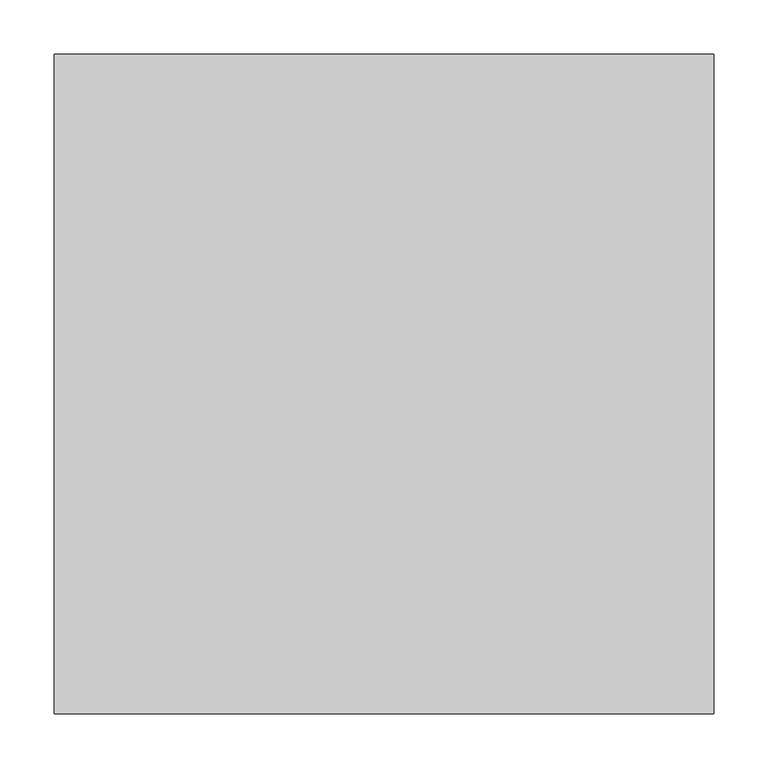
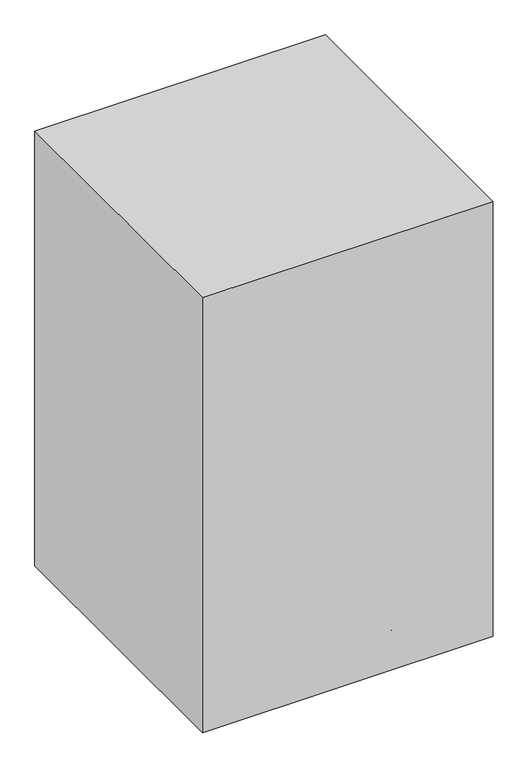
"""IFC4 building model written with IfcOpenShell, lengths in millimetres: proxy geometry, F0340 - Stool, Self Adjusting : F0340 - Stool, Self Adjusting."""

import ifcopenshell
import ifcopenshell.guid

model = None  # the IFC model being written
_history = None  # IfcOwnerHistory: only IFC2X3 demands one
_inside = {}  # id of a spatial element -> (the spatial element, [elements in it])
_under = {}  # id of a project, library or spatial element -> (it, [spatial elements below it])
_declared = {}  # id of a project -> (the project, [libraries it declares])
_typed = {}  # id of a type object -> (the type object, [elements of that type])
_made_of = {}  # id of a material, layer set ... -> (it, [elements and type objects made of it])


def new_model(schema):
    """Start an empty IFC model of exactly this schema.

    Asked for "IFC4X3", IfcOpenShell would pick the latest addendum, in which some entities
    have other attributes; the version numbers below select the first issue.
    IFC2X3 requires an IfcOwnerHistory on every rooted entity: one is made here for all.
    """
    global model, _history
    if schema == "IFC4X3":
        model = ifcopenshell.file(schema_version=(4, 3, 0, 0))
    else:
        model = ifcopenshell.file(schema=schema)
    _inside.clear()
    _under.clear()
    _declared.clear()
    _typed.clear()
    _made_of.clear()
    _history = None
    if model.schema == "IFC2X3":
        org = make("IfcOrganization", Name="unknown")
        user = make(
            "IfcPersonAndOrganization",
            ThePerson=make("IfcPerson", FamilyName="unknown"),
            TheOrganization=org,
        )
        app = make(
            "IfcApplication",
            ApplicationDeveloper=org,
            Version="unknown",
            ApplicationFullName="unknown",
            ApplicationIdentifier="unknown",
        )
        _history = make(
            "IfcOwnerHistory",
            OwningUser=user,
            OwningApplication=app,
            ChangeAction="ADDED",
            CreationDate=0,
        )
    return model


def make(cls, **values):
    """One entity of the class cls with the attributes given. An attribute that is None is left unset."""
    return model.create_entity(
        cls, **{name: value for name, value in values.items() if value is not None}
    )


def rooted(cls, **values):
    """An entity with a GlobalId (a new one), such as an element, a storey or a relation."""
    return make(cls, GlobalId=ifcopenshell.guid.new(), OwnerHistory=_history, **values)


def si_unit(unit_type, name, prefix=None):
    """IfcSIUnit, for example si_unit("LENGTHUNIT", "METRE", prefix="MILLI")."""
    return make("IfcSIUnit", UnitType=unit_type, Prefix=prefix, Name=name)


def assignment(units):
    """IfcUnitAssignment: the units of a project."""
    return None if units is None else make("IfcUnitAssignment", Units=units)


def point(xyz):
    """IfcCartesianPoint."""
    return None if xyz is None else make("IfcCartesianPoint", Coordinates=xyz)


def direction(xyz):
    """IfcDirection."""
    return None if xyz is None else make("IfcDirection", DirectionRatios=xyz)


def frame(location, z_axis=None, x_axis=None):
    """IfcAxis2Placement3D, a coordinate frame: its origin and axes. An axis left out is left unset."""
    return make(
        "IfcAxis2Placement3D",
        Location=point(location),
        Axis=direction(z_axis),
        RefDirection=direction(x_axis),
    )


def frame_2d(location, x_axis=None):
    """IfcAxis2Placement2D, a coordinate frame in the plane: its origin and x axis."""
    return make(
        "IfcAxis2Placement2D", Location=point(location), RefDirection=direction(x_axis)
    )


def origin():
    """The frame at (0, 0, 0) with its axes left unset."""
    return frame((0.0, 0.0, 0.0))


def origin_with_axes():
    """The frame at (0, 0, 0) with the z axis (0, 0, 1) and the x axis (1, 0, 0) written out."""
    return frame((0.0, 0.0, 0.0), z_axis=(0.0, 0.0, 1.0), x_axis=(1.0, 0.0, 0.0))


def origin_2d():
    """The frame at (0, 0) in the plane with its x axis left unset."""
    return frame_2d((0.0, 0.0))


def place(relative_to, where):
    """IfcLocalPlacement: puts the frame where relative to a parent placement (None: the world)."""
    return make(
        "IfcLocalPlacement", PlacementRelTo=relative_to, RelativePlacement=where
    )


def context(
    kind, dimensions, precision=None, world=None, true_north=None, identifier=None
):
    """IfcGeometricRepresentationContext, for example the 3D "Model" context."""
    return make(
        "IfcGeometricRepresentationContext",
        ContextIdentifier=identifier,
        ContextType=kind,
        CoordinateSpaceDimension=dimensions,
        Precision=precision,
        WorldCoordinateSystem=world,
        TrueNorth=true_north,
    )


def project(units=None, contexts=None):
    """IfcProject with its units and contexts."""
    return rooted(
        "IfcProject",
        Name="project",
        RepresentationContexts=contexts,
        UnitsInContext=assignment(units),
    )


def spatial(cls, under=None, at=None, **own):
    """A site, building, storey or space (cls), placed at a placement, below another one or the project."""
    s = rooted(cls, ObjectPlacement=at, **own)
    if under is not None:
        _under.setdefault(under.id(), (under, []))[1].append(s)
    return s


def polyline(points):
    """IfcPolyline through the points."""
    return make("IfcPolyline", Points=[point(p) for p in points])


def circle_curve(where, radius):
    """IfcCircle in the frame where."""
    return make("IfcCircle", Position=where, Radius=radius)


def trimmed(basis, trim1, trim2, sense, master):
    """IfcTrimmedCurve: the piece of a basis curve between two trims."""
    return make(
        "IfcTrimmedCurve",
        BasisCurve=basis,
        Trim1=trim1,
        Trim2=trim2,
        SenseAgreement=sense,
        MasterRepresentation=master,
    )


def segment(curve, same_sense, transition):
    """IfcCompositeCurveSegment."""
    return make(
        "IfcCompositeCurveSegment",
        Transition=transition,
        SameSense=same_sense,
        ParentCurve=curve,
    )


def composite_curve(segments, self_intersect=None):
    """IfcCompositeCurve: segments joined end to end."""
    return make("IfcCompositeCurve", Segments=segments, SelfIntersect=self_intersect)


def outline(outer, holes=None, kind="AREA"):
    """IfcArbitraryClosedProfileDef: a profile drawn as a closed curve; with holes, ...WithVoids."""
    if holes is None:
        return make("IfcArbitraryClosedProfileDef", ProfileType=kind, OuterCurve=outer)
    return make(
        "IfcArbitraryProfileDefWithVoids",
        ProfileType=kind,
        OuterCurve=outer,
        InnerCurves=holes,
    )


def extrude(swept, where, along, depth):
    """IfcExtrudedAreaSolid: the profile swept, set in the frame where, extruded along a direction by depth."""
    return make(
        "IfcExtrudedAreaSolid",
        SweptArea=swept,
        Position=where,
        ExtrudedDirection=direction(along),
        Depth=depth,
    )


def shape(context_of_items, identifier, shape_type, items):
    """IfcShapeRepresentation: the items that make up one representation, for example the "Body"."""
    return make(
        "IfcShapeRepresentation",
        ContextOfItems=context_of_items,
        RepresentationIdentifier=identifier,
        RepresentationType=shape_type,
        Items=items,
    )


def source(mapping_origin, context_of_items, identifier, shape_type, items):
    """IfcRepresentationMap: a shape defined once, which mapped items show again and again."""
    return make(
        "IfcRepresentationMap",
        MappingOrigin=mapping_origin,
        MappedRepresentation=shape(context_of_items, identifier, shape_type, items),
    )


def transform(
    local_origin,
    x_axis=None,
    y_axis=None,
    z_axis=None,
    scale=None,
    scale2=None,
    scale3=None,
    uniform=True,
):
    """IfcCartesianTransformationOperator3D, or its non-uniform kind. x_axis, y_axis, z_axis: its Axis1, 2, 3."""
    if uniform:
        return make(
            "IfcCartesianTransformationOperator3D",
            Axis1=direction(x_axis),
            Axis2=direction(y_axis),
            LocalOrigin=point(local_origin),
            Scale=scale,
            Axis3=direction(z_axis),
        )
    return make(
        "IfcCartesianTransformationOperator3DnonUniform",
        Axis1=direction(x_axis),
        Axis2=direction(y_axis),
        LocalOrigin=point(local_origin),
        Scale=scale,
        Axis3=direction(z_axis),
        Scale2=scale2,
        Scale3=scale3,
    )


def mapped(mapping_source, mapping_target):
    """IfcMappedItem: shows the shape of a source again, moved by a transform."""
    return make(
        "IfcMappedItem", MappingSource=mapping_source, MappingTarget=mapping_target
    )


def made_of(thing, what):
    """Note that an element or type object is made of a material, layer set ...; save() writes the relation."""
    if what is not None:
        _made_of.setdefault(what.id(), (what, []))[1].append(thing)
    return thing


def element(
    cls,
    number,
    at=None,
    inside=None,
    cuts=None,
    type_object=None,
    material=None,
    context=None,
    identifier="Body",
    shape_type=None,
    held_by="IfcProductDefinitionShape",
    body=None,
    shapes=None,
    **own,
):
    """One element of the class cls, such as IfcWall. Its Tag is "e" and its number.

    at: its placement. inside: the storey or other place that contains it. cuts: it is an
    opening in that element (IfcRelVoidsElement). A single representation is given by context,
    identifier, shape_type and body (its items); several are given by shapes. held_by: the class
    of the entity that holds the representations. save() writes the other relations.
    """
    e = rooted(cls, Tag="e%d" % number, ObjectPlacement=at, **own)
    if body is not None:
        shapes = [shape(context, identifier, shape_type, body)]
    if shapes is not None:
        e.Representation = make(held_by, Representations=shapes)
    if inside is not None:
        _inside.setdefault(inside.id(), (inside, []))[1].append(e)
    if cuts is not None:
        rooted(
            "IfcRelVoidsElement", RelatingBuildingElement=cuts, RelatedOpeningElement=e
        )
    if type_object is not None:
        _typed.setdefault(type_object.id(), (type_object, []))[1].append(e)
    return made_of(e, material)


def aggregate(whole, parts):
    """IfcRelAggregates: a whole, such as a stair, and the parts it consists of."""
    return rooted("IfcRelAggregates", RelatingObject=whole, RelatedObjects=parts)


def save(model, path):
    """Write the relations noted so far, then the file.

    IfcRelAggregates (storeys below a building ...), IfcRelContainedInSpatialStructure (elements
    in a storey), IfcRelDefinesByType, IfcRelAssociatesMaterial and IfcRelDeclares: one each for
    every whole, place, type object, material and project.
    """
    for whole, parts in _under.values():
        aggregate(whole, parts)
    for where, things in _inside.values():
        rooted(
            "IfcRelContainedInSpatialStructure",
            RelatedElements=things,
            RelatingStructure=where,
        )
    for kind, things in _typed.values():
        rooted("IfcRelDefinesByType", RelatedObjects=things, RelatingType=kind)
    for what, things in _made_of.values():
        rooted("IfcRelAssociatesMaterial", RelatedObjects=things, RelatingMaterial=what)
    for by, libraries in _declared.values():
        rooted("IfcRelDeclares", RelatingContext=by, RelatedDefinitions=libraries)
    model.write(path)


def specialty_equipment_6f838b8f(model_context):
    return source(origin(), model_context, "Body", "SweptSolid", [
        extrude(outline(composite_curve([segment(trimmed(circle_curve(frame_2d((0.0, -25.7612183)), 25.7612183), [point((0.0, -51.5224365))], [point((0.0, 0.0))], False, "CARTESIAN"), True, "CONTINUOUS"), segment(trimmed(circle_curve(frame_2d((0.0, -25.7612183)), 25.7612183), [point((0.0, 0.0))], [point((0.0, -51.5224365))], False, "CARTESIAN"), True, "CONTINUOUS")], self_intersect=False)), frame((203.8559823, 49.544861, 25.7612183), z_axis=(-0.3090169943748919, 0.9510565162951716, 0.0), x_axis=(0.0, 0.0, -1.0)), (0.0, 0.0, 1.0), 31.75),
        extrude(outline(composite_curve([segment(polyline([(-57.1058784, 0.0), (-0.678315, 0.0)]), True, "CONTINUOUS"), segment(trimmed(circle_curve(frame_2d((-28.8920968, 0.0)), 28.2137817), [point((-0.678315, 0.0))], [point((-57.1058784, 0.0))], False, "CARTESIAN"), True, "CONTINUOUS")], self_intersect=False)), frame((256.8155026, 63.4140597, 25.7612183), z_axis=(-0.30901699437489183, 0.9510565162951716, 0.0), x_axis=(0.9510565162951716, 0.30901699437489183, 0.0)), (0.0, 0.0, 1.0), 38.1),
        extrude(outline(composite_curve([segment(trimmed(circle_curve(frame_2d((223.4509477, 72.6028121)), 3.5091751), [point((222.3665529, 75.940236))], [point((224.5353424, 69.2653883))], False, "CARTESIAN"), True, "CONTINUOUS"), segment(trimmed(circle_curve(frame_2d((223.4509477, 72.6028121)), 3.5091751), [point((224.5353424, 69.2653883))], [point((222.3665529, 75.940236))], False, "CARTESIAN"), True, "CONTINUOUS")], self_intersect=False)), frame((0.0, 0.0, 53.975), z_axis=(0.0, 0.0, 1.0), x_axis=(1.0, 0.0, 0.0)), (0.0, 0.0, 1.0), 13.49375),
        extrude(outline(polyline([(230.0293313, 68.0638809), (25.3978935, 1.5750963), (21.4736172, 13.6527769), (226.105055, 80.1415615), (230.0293313, 68.0638809)])), frame((0.0, 0.0, 67.46875), z_axis=(0.0, 0.0, 1.0), x_axis=(1.0, 0.0, 0.0)), (0.0, 0.0, 1.0), 50.8),
        extrude(outline(composite_curve([segment(trimmed(circle_curve(frame_2d((0.0, -25.7612182)), 25.7612183), [point((0.0, -51.5224365))], [point((0.0, 0.0))], False, "CARTESIAN"), True, "CONTINUOUS"), segment(trimmed(circle_curve(frame_2d((0.0, -25.7612182)), 25.7612183), [point((0.0, 0.0))], [point((0.0, -51.5224365))], False, "CARTESIAN"), True, "CONTINUOUS")], self_intersect=False)), frame((110.1149259, -178.5683563, 25.7612183), z_axis=(0.8090169943749846, 0.5877852522924221, 0.0), x_axis=(0.0, 0.0, -1.0)), (0.0, 0.0, 1.0), 31.75),
        extrude(outline(composite_curve([segment(polyline([(-57.1058785, 0.0), (-0.6783149, 0.0)]), True, "CONTINUOUS"), segment(trimmed(circle_curve(frame_2d((-28.8920966, 0.0)), 28.2137817), [point((-0.6783149, 0.0))], [point((-57.1058785, 0.0))], False, "CARTESIAN"), True, "CONTINUOUS")], self_intersect=False)), frame((139.6707094, -224.6500351, 25.7612183), z_axis=(0.8090169943749845, 0.5877852522924222, 0.0), x_axis=(0.5877852522924222, -0.8090169943749845, 0.0)), (0.0, 0.0, 1.0), 38.1),
        extrude(outline(composite_curve([segment(trimmed(circle_curve(frame_2d((138.0995178, -190.0789771)), 3.5091751), [point((140.9385001, -188.0163357))], [point((135.2605355, -192.1416185))], False, "CARTESIAN"), True, "CONTINUOUS"), segment(trimmed(circle_curve(frame_2d((138.0995178, -190.0789771)), 3.5091751), [point((135.2605355, -192.1416185))], [point((140.9385001, -188.0163357))], False, "CARTESIAN"), True, "CONTINUOUS")], self_intersect=False)), frame((0.0, 0.0, 53.975), z_axis=(0.0, 0.0, 1.0), x_axis=(1.0, 0.0, 0.0)), (0.0, 0.0, 1.0), 13.49375),
        extrude(outline(polyline([(135.81557, -197.7379985), (9.3463863, -23.6681006), (19.620275, -16.2036835), (146.0894588, -190.2735815), (135.81557, -197.7379985)])), frame((0.0, 0.0, 67.46875), z_axis=(0.0, 0.0, 1.0), x_axis=(1.0, 0.0, 0.0)), (0.0, 0.0, 1.0), 50.8),
        extrude(outline(composite_curve([segment(trimmed(circle_curve(frame_2d((0.0, -25.7612182)), 25.7612183), [point((0.0, -51.5224365))], [point((0.0, 0.0))], False, "CARTESIAN"), True, "CONTINUOUS"), segment(trimmed(circle_curve(frame_2d((0.0, -25.7612182)), 25.7612183), [point((0.0, 0.0))], [point((0.0, -51.5224365))], False, "CARTESIAN"), True, "CONTINUOUS")], self_intersect=False)), frame((-110.1149259, -178.5683563, 25.7612183), z_axis=(-0.8090169943749151, 0.5877852522925178, 0.0), x_axis=(0.0, 0.0, 1.0)), (0.0, 0.0, 1.0), 31.75),
        extrude(outline(composite_curve([segment(trimmed(circle_curve(frame_2d((28.8920966, 0.0)), 28.2137817), [point((57.1058785, 0.0))], [point((0.6783149, 0.0))], False, "CARTESIAN"), True, "CONTINUOUS"), segment(polyline([(0.6783149, 0.0), (57.1058785, 0.0)]), True, "CONTINUOUS")], self_intersect=False)), frame((-139.6707094, -224.6500351, 25.7612183), z_axis=(-0.809016994374915, 0.5877852522925177, 0.0), x_axis=(0.5877852522925177, 0.809016994374915, 0.0)), (0.0, 0.0, 1.0), 38.1),
        extrude(outline(composite_curve([segment(trimmed(circle_curve(frame_2d((-138.1007518, -190.0780805)), 3.5091751), [point((-135.2617695, -192.1407219))], [point((-140.9397341, -188.0154391))], False, "CARTESIAN"), True, "CONTINUOUS"), segment(trimmed(circle_curve(frame_2d((-138.1007518, -190.0780805)), 3.5091751), [point((-140.9397341, -188.0154391))], [point((-135.2617695, -192.1407219))], False, "CARTESIAN"), True, "CONTINUOUS")], self_intersect=False)), frame((0.0, 0.0, 53.975), z_axis=(0.0, 0.0, 1.0), x_axis=(1.0, 0.0, 0.0)), (0.0, 0.0, 1.0), 13.49375),
        extrude(outline(polyline([(-146.0906928, -190.2726849), (-19.6215091, -16.2027869), (-9.3476203, -23.667204), (-135.8168041, -197.737102), (-146.0906928, -190.2726849)])), frame((0.0, 0.0, 67.46875), z_axis=(0.0, 0.0, 1.0), x_axis=(1.0, 0.0, 0.0)), (0.0, 0.0, 1.0), 50.8),
        extrude(outline(composite_curve([segment(trimmed(circle_curve(frame_2d((0.0, -25.7612183)), 25.7612183), [point((0.0, -51.5224365))], [point((0.0, 0.0))], False, "CARTESIAN"), True, "CONTINUOUS"), segment(trimmed(circle_curve(frame_2d((0.0, -25.7612183)), 25.7612183), [point((0.0, 0.0))], [point((0.0, -51.5224365))], False, "CARTESIAN"), True, "CONTINUOUS")], self_intersect=False)), frame((-203.8559823, 49.544861, 25.7612183), z_axis=(0.3090169943749793, 0.9510565162951433, 0.0), x_axis=(0.0, 0.0, 1.0)), (0.0, 0.0, 1.0), 31.75),
        extrude(outline(composite_curve([segment(trimmed(circle_curve(frame_2d((28.8920968, 0.0)), 28.2137817), [point((57.1058784, 0.0))], [point((0.678315, 0.0))], False, "CARTESIAN"), True, "CONTINUOUS"), segment(polyline([(0.678315, 0.0), (57.1058784, 0.0)]), True, "CONTINUOUS")], self_intersect=False)), frame((-256.8155026, 63.4140597, 25.7612183), z_axis=(0.3090169943749793, 0.9510565162951433, 0.0), x_axis=(0.9510565162951433, -0.3090169943749793, 0.0)), (0.0, 0.0, 1.0), 38.1),
        extrude(outline(composite_curve([segment(trimmed(circle_curve(frame_2d((-223.4504763, 72.6042628)), 3.5091751), [point((-224.5348711, 69.266839))], [point((-222.3660816, 75.9416867))], False, "CARTESIAN"), True, "CONTINUOUS"), segment(trimmed(circle_curve(frame_2d((-223.4504763, 72.6042628)), 3.5091751), [point((-222.3660816, 75.9416867))], [point((-224.5348711, 69.266839))], False, "CARTESIAN"), True, "CONTINUOUS")], self_intersect=False)), frame((0.0, 0.0, 53.975), z_axis=(0.0, 0.0, 1.0), x_axis=(1.0, 0.0, 0.0)), (0.0, 0.0, 1.0), 13.49375),
        extrude(outline(polyline([(-226.1045836, 80.1430121), (-21.4731458, 13.6542275), (-25.3974221, 1.576547), (-230.0288599, 68.0653316), (-226.1045836, 80.1430121)])), frame((0.0, 0.0, 67.46875), z_axis=(0.0, 0.0, 1.0), x_axis=(1.0, 0.0, 0.0)), (0.0, 0.0, 1.0), 50.8),
        extrude(outline(composite_curve([segment(trimmed(circle_curve(frame_2d((234.9499827, 25.7612183)), 25.7612183), [point((260.7112009, 25.7612183))], [point((209.1887644, 25.7612183))], False, "CARTESIAN"), True, "CONTINUOUS"), segment(trimmed(circle_curve(frame_2d((234.9499827, 25.7612183)), 25.7612183), [point((209.1887644, 25.7612183))], [point((260.7112009, 25.7612183))], False, "CARTESIAN"), True, "CONTINUOUS")], self_intersect=False)), frame((-15.875, 0.0, 0.0), z_axis=(1.0, 0.0, 0.0), x_axis=(0.0, 1.0, 0.0)), (0.0, 0.0, 1.0), 31.75),
        extrude(outline(composite_curve([segment(trimmed(circle_curve(frame_2d((234.9499827, 25.7612183)), 28.2137817), [point((206.7362009, 25.7612183))], [point((263.1637644, 25.7612183))], False, "CARTESIAN"), True, "CONTINUOUS"), segment(polyline([(263.1637644, 25.7612183), (206.7362009, 25.7612183)]), True, "CONTINUOUS")], self_intersect=False)), frame((-19.05, 0.0, 0.0), z_axis=(1.0, 0.0, 0.0), x_axis=(0.0, 1.0, 0.0)), (0.0, 0.0, 1.0), 38.1),
        extrude(outline(composite_curve([segment(trimmed(circle_curve(frame_2d((0.0007627, 234.9499827)), 3.5091751), [point((-3.5084124, 234.9499827))], [point((3.5099378, 234.9499827))], False, "CARTESIAN"), True, "CONTINUOUS"), segment(trimmed(circle_curve(frame_2d((0.0007627, 234.9499827)), 3.5091751), [point((3.5099378, 234.9499827))], [point((-3.5084124, 234.9499827))], False, "CARTESIAN"), True, "CONTINUOUS")], self_intersect=False)), frame((0.0, 0.0, 53.975), z_axis=(0.0, 0.0, 1.0), x_axis=(1.0, 0.0, 0.0)), (0.0, 0.0, 1.0), 13.49375),
        extrude(outline(polyline([(6.3503751, 239.8037904), (6.3503751, 24.6415636), (-6.3488498, 24.6415636), (-6.3488498, 239.8037904), (6.3503751, 239.8037904)])), frame((0.0, 0.0, 67.46875), z_axis=(0.0, 0.0, 1.0), x_axis=(1.0, 0.0, 0.0)), (0.0, 0.0, 1.0), 50.8),
        extrude(outline(composite_curve([segment(trimmed(circle_curve(origin_2d(), 25.4466483), [point((-25.4466483, 0.0))], [point((25.4466483, 0.0))], False, "CARTESIAN"), True, "CONTINUOUS"), segment(trimmed(circle_curve(origin_2d(), 25.4466483), [point((25.4466483, 0.0))], [point((-25.4466483, 0.0))], False, "CARTESIAN"), True, "CONTINUOUS")], self_intersect=False)), frame((0.0, 0.0, 67.46875), z_axis=(0.0, 0.0, 1.0), x_axis=(1.0, 0.0, 0.0)), (0.0, 0.0, 1.0), 542.13125),
        extrude(outline(composite_curve([segment(trimmed(circle_curve(origin_2d(), 254.0), [point((-254.0, 0.0))], [point((254.0, 0.0))], False, "CARTESIAN"), True, "CONTINUOUS"), segment(trimmed(circle_curve(origin_2d(), 254.0), [point((254.0, 0.0))], [point((-254.0, 0.0))], False, "CARTESIAN"), True, "CONTINUOUS")], self_intersect=False)), frame((0.0, 0.0, 609.6), z_axis=(0.0, 0.0, 1.0), x_axis=(1.0, 0.0, 0.0)), (0.0, 0.0, 1.0), 50.8),
        extrude(outline(polyline([(304.8, 304.8), (304.8, -304.8), (-304.8, -304.8), (-304.8, 304.8), (304.8, 304.8)])), origin_with_axes(), (0.0, 0.0, 1.0), 965.2),
    ])


if __name__ == "__main__":
    model = new_model("IFC4")
    model_context = context("Model", 3, world=origin())
    ifc_project = project(units=[si_unit("LENGTHUNIT", "METRE", prefix="MILLI")], contexts=[model_context])
    site = spatial("IfcSite", under=ifc_project)
    building = spatial("IfcBuilding", under=site)
    placement = place(None, origin())
    specialty_equipment_shape = specialty_equipment_6f838b8f(model_context)
    element("IfcBuildingElementProxy", 1, Name="F0340 - Stool, Self Adjusting : F0340 - Stool, Self Adjusting", ObjectType="F0340 - Stool, Self Adjusting : F0340 - Stool, Self Adjusting", at=placement, inside=building, context=model_context, shape_type="MappedRepresentation", body=[
        mapped(specialty_equipment_shape, transform((0.0, 0.0, 0.0), x_axis=(1.0, 0.0, 0.0), y_axis=(0.0, 1.0, 0.0), z_axis=(0.0, 0.0, 1.0))),
    ])
    save(model, "model.ifc")

# Revit data of these elements
# Type "F0340 - Stool, Self Adjusting : F0340 - Stool, Self Adjusting"
#   Watts2 = "0"
#   Watts1 = "0"
#   Unit_Issue = "EA"
#   UTIL_6_Misc = "-"
#   UTIL_5_NonMedGas = "-"
#   UTIL_4_MiscGas = "-"
#   UTIL_3_MedGas = "-"
#   UTIL_2_Elec = "-"
#   UTIL_1_WaterDrain = "-"
#   Nomenclature = "Stool, Self Adjusting"
#   NSN = "6530"
#   Location [instance default] = ""
#   JSN = "F0340"
#   Fund_Source_VA = "-"
#   Fund_Source_Navy = "-"
#   Fund_Source_Army = "-"
#   Fund_Source_AF = "-"
#   ELEC_Volts2 = "0"
#   ELEC_Volts1 = "0"
#   ELEC_Phase2 = "0"
#   ELEC_Phase1 = "0"
#   ELEC_HertzSwitch = "0"
#   ELEC_HertzDependent = "0"
#   ELEC_Hertz = "0"
#   ELEC_Amps2 = "0"
#   ELEC_Amps1 = "0"
#   DetailDescription = "Self adjusting stool. Consists of a foam padded upholstered seat with attached foot rest for added comfort. Mounted on swivel casters.  Designed for doctor''s use during examinations."
#   CAT_VA = "C"
#   CAT_Navy = "C"
#   CAT_IHS = "-"
#   CAT_Army = "C"
#   CAT_AF = "C"
#   BTUperhour = "0"
#   Weight_IP = 39
#   DIM_Width_IP = 2' - 0"
#   DIM_Height_IP = 3' - 2"
#   DIM_Depth_IP = 2' - 0"
#   Assembly Code = ""
# Element 1 (IfcBuildingElementProxy, "F0340 - Stool, Self Adjusting : F0340 - Stool, Self Adjusting")
#   Materials on its faces: "Stool metal", "Stool caster", "EquipSpace", "Stool cushion"
# Materials
#   "Stool metal": class "Unassigned", colour RGB 201 201 201, transparency 0, Comments = "Rendering appearance not upgraded "
#   "Stool caster": class "Unassigned", colour RGB 0 0 0, transparency 0, Comments = "Rendering appearance not upgraded "
#   "EquipSpace": class "Unassigned", colour RGB 221 217 195, transparency 0.5
#   "Stool cushion": class "Unassigned", colour RGB 226 128 109, transparency 0, Comments = "Rendering appearance not upgraded "
